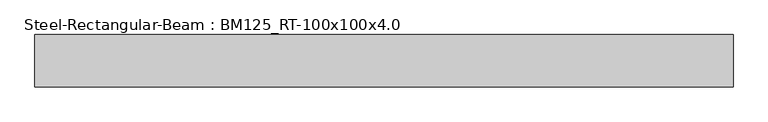
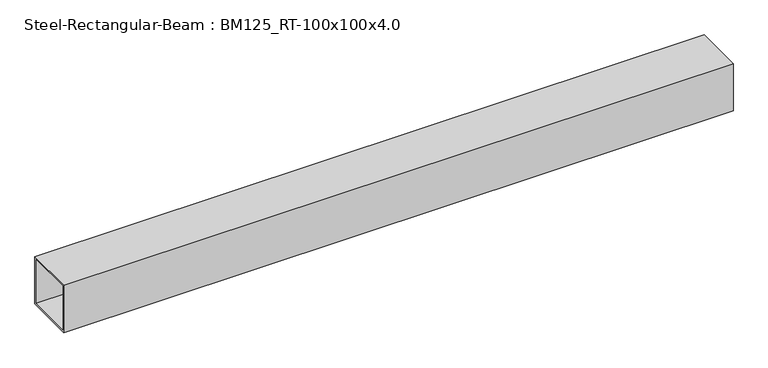
"""IFC4 building model written with IfcOpenShell, lengths in millimetres: beam geometry, Steel-Rectangular-Beam : BM125_RT-100x100x4.0."""

from ifc_helpers import new_model, si_unit, frame, origin, place, context, project, spatial, polyline, outline, extrude, source, transform, mapped, element, save


def steel_rectangular_beam_bm125_rt_100x100x4_0_d4cde651(model_context):
    return source(origin(), model_context, "Body", "SweptSolid", [
        extrude(outline(polyline([(-50.0, 50.0), (50.0, 50.0), (50.0, -50.0), (-50.0, -50.0), (-50.0, 50.0)]), holes=[polyline([(46.0, -46.0), (46.0, 46.0), (-46.0, 46.0), (-46.0, -46.0), (46.0, -46.0)])]), frame((-612.3, 0.0, 0.0), z_axis=(1.0, 0.0, 0.0), x_axis=(0.0, 1.0, 0.0)), (0.0, 0.0, 1.0), 1337.3),
        extrude(outline(polyline([(-50.0, 50.0), (50.0, 50.0), (50.0, -50.0), (-50.0, -50.0), (-50.0, 50.0)]), holes=[polyline([(46.0, -46.0), (46.0, 46.0), (-46.0, 46.0), (-46.0, -46.0), (46.0, -46.0)])]), frame((-612.3, 0.0, 0.0), z_axis=(1.0, 0.0, 0.0), x_axis=(0.0, 1.0, 0.0)), (0.0, 0.0, 1.0), 1337.3),
        extrude(outline(polyline([(-50.0, 50.0), (50.0, 50.0), (50.0, -50.0), (-50.0, -50.0), (-50.0, 50.0)]), holes=[polyline([(46.0, -46.0), (46.0, 46.0), (-46.0, 46.0), (-46.0, -46.0), (46.0, -46.0)])]), frame((-612.3, 0.0, 0.0), z_axis=(1.0, 0.0, 0.0), x_axis=(0.0, 1.0, 0.0)), (0.0, 0.0, 1.0), 1337.3),
        extrude(outline(polyline([(-50.0, 50.0), (50.0, 50.0), (50.0, -50.0), (-50.0, -50.0), (-50.0, 50.0)]), holes=[polyline([(46.0, -46.0), (46.0, 46.0), (-46.0, 46.0), (-46.0, -46.0), (46.0, -46.0)])]), frame((-612.3, 0.0, 0.0), z_axis=(1.0, 0.0, 0.0), x_axis=(0.0, 1.0, 0.0)), (0.0, 0.0, 1.0), 1337.3),
    ])


if __name__ == "__main__":
    model = new_model("IFC4")
    model_context = context("Model", 3, world=origin())
    ifc_project = project(units=[si_unit("LENGTHUNIT", "METRE", prefix="MILLI")], contexts=[model_context])
    site = spatial("IfcSite", under=ifc_project)
    building = spatial("IfcBuilding", under=site)
    placement = place(None, origin())
    steel_rectangular_beam_bm125_rt_100x100x4_0_shape = steel_rectangular_beam_bm125_rt_100x100x4_0_d4cde651(model_context)
    element("IfcBeam", 1, ObjectType="Steel-Rectangular-Beam : BM125_RT-100x100x4.0", at=placement, inside=building, context=model_context, shape_type="MappedRepresentation", body=[
        mapped(steel_rectangular_beam_bm125_rt_100x100x4_0_shape, transform((0.0, 0.0, 0.0), x_axis=(1.0, 0.0, 0.0), y_axis=(0.0, 1.0, 0.0), z_axis=(0.0, 0.0, 1.0))),
    ])
    save(model, "model.ifc")

# Revit data of these elements
# Type "Steel-Rectangular-Beam : BM125_RT-100x100x4.0"
#   t = 4 mm
#   Mass per Unit Length = 11.70 kg/m
#   Surface Area = 0.386 m²/m
#   Sectional Area = 14.95 cm²
#   Length [instance default] = 3000 mm
#   H = 100 mm
#   B = 100 mm
#   hec_material4 [instance default] = none
#   hec_material3 [instance default] = none
#   hec_material2 [instance default] = none
#   hec_material1 [instance default] = none
#   Structural Material [instance default] = none
# Element 1 (IfcBeam, "Steel-Rectangular-Beam : BM125_RT-100x100x4.0")
#   hec_material2 = S01AA010-00001_Main Steel Structure Fabrication Work_Shelter/Building_Steel Painting/Coating_for Non-Fireproofed Steel Surface, Surface Preparation, Primer, Second & Final Coat
#   hec_material1 = S03AA007-00001_Main Steel Structure Erection Work_Girth & Purlin
#   Structural Material = S01AA007-00001_Main Steel Structure Fabrication Work_Shelter/Building_Girth & Purlin
#   Materials on its faces: "S01AA010-00001_Main Steel Structure Fabrication Work_Shelter/Building_Steel Painting/Coating_for Non-Fireproofed Steel Surface, Surface Preparation, Primer, Second & Final Coat"
# Materials
#   "S01AA010-00001_Main Steel Structure Fabrication Work_Shelter/Building_Steel Painting/Coating_for Non-Fireproofed Steel Surface, Surface Preparation, Primer, Second & Final Coat": class "Metal", colour RGB 120 120 120, transparency 0, Description = "Paint finished steel", W00) Work Master Code = "S01AA010-00001", W01) Work Master_Lv1 = "Main Steel Structure Fabrication Work", W02) Work Master_Lv2 = "Shelter/Building", W03) Work Master_Spec.1 = "Steel Painting/Coating", W04) Work Master_Spec.2 = "for Non-Fireproofed Steel Surface, Surface Preparation, Primer, Second & Final Coat", Cost = 0
#   "S03AA007-00001_Main Steel Structure Erection Work_Girth & Purlin": class "Metal", colour RGB 120 120 120, transparency 0, Comments = "(30KG/M>Weight)", Description = "Structural steel 50ksi", W00) Work Master Code = "S03AA007-00001", W01) Work Master_Lv1 = "Main Steel Structure Erection Work", W02) Work Master_Lv2 = "Shelter/Building", W03) Work Master_Spec.1 = "Girth & Purlin", Cost = 0
#   "S01AA007-00001_Main Steel Structure Fabrication Work_Shelter/Building_Girth & Purlin": class "Metal", colour RGB 120 120 120, transparency 0, Comments = "(30KG/M>Weight)", Description = "Structural steel 50ksi", W00) Work Master Code = "S01AA007-00001", W01) Work Master_Lv1 = "Main Steel Structure Fabrication Work", W02) Work Master_Lv2 = "Shelter/Building", W03) Work Master_Spec.1 = "Girth & Purlin", Cost = 0
